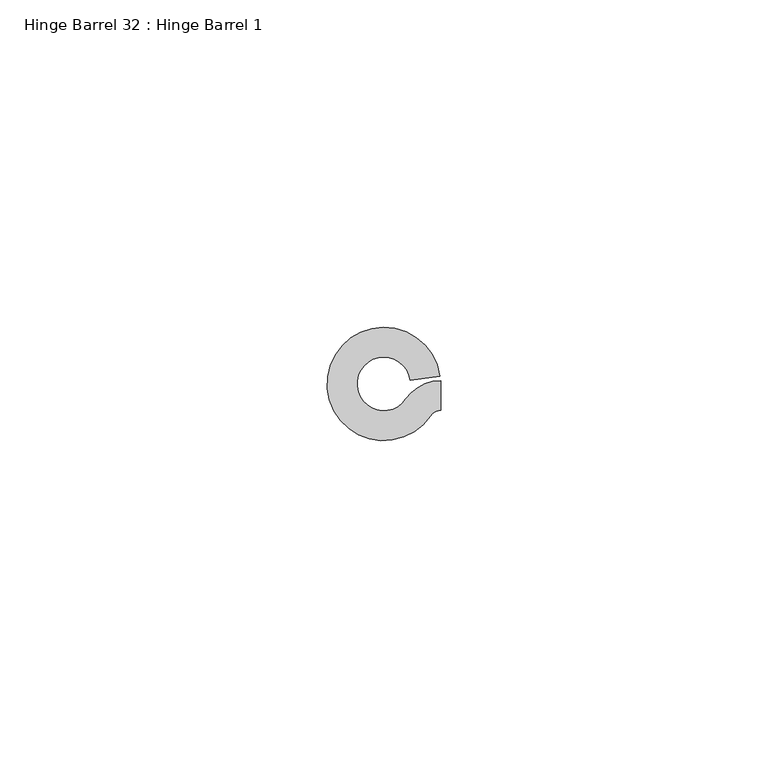
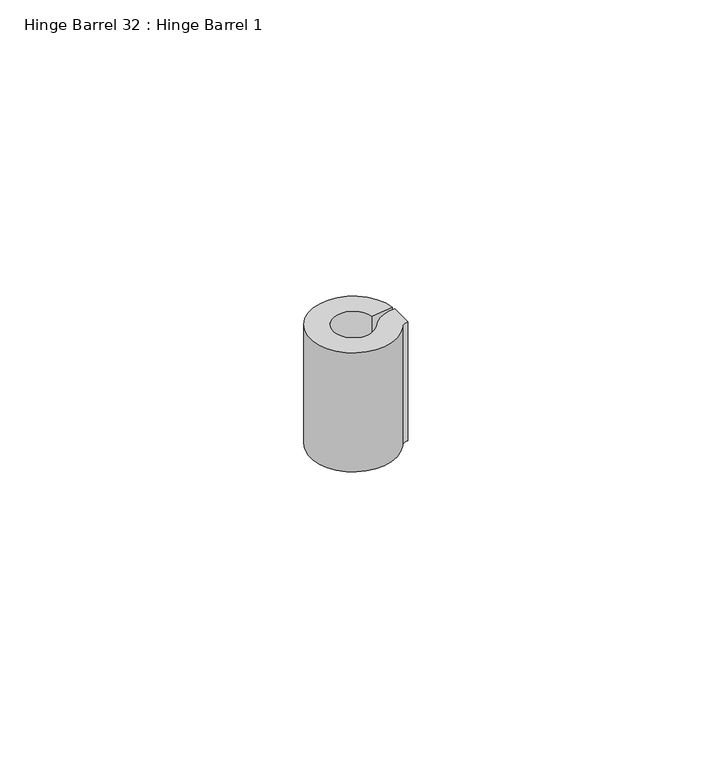
"""IFC4 building model written with IfcOpenShell, lengths in millimetres: proxy geometry, Hinge Barrel 32 : Hinge Barrel 1."""

import ifcopenshell
import ifcopenshell.guid

model = None  # the IFC model being written
_history = None  # IfcOwnerHistory: only IFC2X3 demands one
_inside = {}  # id of a spatial element -> (the spatial element, [elements in it])
_under = {}  # id of a project, library or spatial element -> (it, [spatial elements below it])
_declared = {}  # id of a project -> (the project, [libraries it declares])
_typed = {}  # id of a type object -> (the type object, [elements of that type])
_made_of = {}  # id of a material, layer set ... -> (it, [elements and type objects made of it])


def new_model(schema):
    """Start an empty IFC model of exactly this schema.

    Asked for "IFC4X3", IfcOpenShell would pick the latest addendum, in which some entities
    have other attributes; the version numbers below select the first issue.
    IFC2X3 requires an IfcOwnerHistory on every rooted entity: one is made here for all.
    """
    global model, _history
    if schema == "IFC4X3":
        model = ifcopenshell.file(schema_version=(4, 3, 0, 0))
    else:
        model = ifcopenshell.file(schema=schema)
    _inside.clear()
    _under.clear()
    _declared.clear()
    _typed.clear()
    _made_of.clear()
    _history = None
    if model.schema == "IFC2X3":
        org = make("IfcOrganization", Name="unknown")
        user = make(
            "IfcPersonAndOrganization",
            ThePerson=make("IfcPerson", FamilyName="unknown"),
            TheOrganization=org,
        )
        app = make(
            "IfcApplication",
            ApplicationDeveloper=org,
            Version="unknown",
            ApplicationFullName="unknown",
            ApplicationIdentifier="unknown",
        )
        _history = make(
            "IfcOwnerHistory",
            OwningUser=user,
            OwningApplication=app,
            ChangeAction="ADDED",
            CreationDate=0,
        )
    return model


def make(cls, **values):
    """One entity of the class cls with the attributes given. An attribute that is None is left unset."""
    return model.create_entity(
        cls, **{name: value for name, value in values.items() if value is not None}
    )


def rooted(cls, **values):
    """An entity with a GlobalId (a new one), such as an element, a storey or a relation."""
    return make(cls, GlobalId=ifcopenshell.guid.new(), OwnerHistory=_history, **values)


def si_unit(unit_type, name, prefix=None):
    """IfcSIUnit, for example si_unit("LENGTHUNIT", "METRE", prefix="MILLI")."""
    return make("IfcSIUnit", UnitType=unit_type, Prefix=prefix, Name=name)


def assignment(units):
    """IfcUnitAssignment: the units of a project."""
    return None if units is None else make("IfcUnitAssignment", Units=units)


def point(xyz):
    """IfcCartesianPoint."""
    return None if xyz is None else make("IfcCartesianPoint", Coordinates=xyz)


def direction(xyz):
    """IfcDirection."""
    return None if xyz is None else make("IfcDirection", DirectionRatios=xyz)


def frame(location, z_axis=None, x_axis=None):
    """IfcAxis2Placement3D, a coordinate frame: its origin and axes. An axis left out is left unset."""
    return make(
        "IfcAxis2Placement3D",
        Location=point(location),
        Axis=direction(z_axis),
        RefDirection=direction(x_axis),
    )


def frame_2d(location, x_axis=None):
    """IfcAxis2Placement2D, a coordinate frame in the plane: its origin and x axis."""
    return make(
        "IfcAxis2Placement2D", Location=point(location), RefDirection=direction(x_axis)
    )


def origin():
    """The frame at (0, 0, 0) with its axes left unset."""
    return frame((0.0, 0.0, 0.0))


def place(relative_to, where):
    """IfcLocalPlacement: puts the frame where relative to a parent placement (None: the world)."""
    return make(
        "IfcLocalPlacement", PlacementRelTo=relative_to, RelativePlacement=where
    )


def context(
    kind, dimensions, precision=None, world=None, true_north=None, identifier=None
):
    """IfcGeometricRepresentationContext, for example the 3D "Model" context."""
    return make(
        "IfcGeometricRepresentationContext",
        ContextIdentifier=identifier,
        ContextType=kind,
        CoordinateSpaceDimension=dimensions,
        Precision=precision,
        WorldCoordinateSystem=world,
        TrueNorth=true_north,
    )


def project(units=None, contexts=None):
    """IfcProject with its units and contexts."""
    return rooted(
        "IfcProject",
        Name="project",
        RepresentationContexts=contexts,
        UnitsInContext=assignment(units),
    )


def spatial(cls, under=None, at=None, **own):
    """A site, building, storey or space (cls), placed at a placement, below another one or the project."""
    s = rooted(cls, ObjectPlacement=at, **own)
    if under is not None:
        _under.setdefault(under.id(), (under, []))[1].append(s)
    return s


def polyline(points):
    """IfcPolyline through the points."""
    return make("IfcPolyline", Points=[point(p) for p in points])


def circle_curve(where, radius):
    """IfcCircle in the frame where."""
    return make("IfcCircle", Position=where, Radius=radius)


def trimmed(basis, trim1, trim2, sense, master):
    """IfcTrimmedCurve: the piece of a basis curve between two trims."""
    return make(
        "IfcTrimmedCurve",
        BasisCurve=basis,
        Trim1=trim1,
        Trim2=trim2,
        SenseAgreement=sense,
        MasterRepresentation=master,
    )


def segment(curve, same_sense, transition):
    """IfcCompositeCurveSegment."""
    return make(
        "IfcCompositeCurveSegment",
        Transition=transition,
        SameSense=same_sense,
        ParentCurve=curve,
    )


def composite_curve(segments, self_intersect=None):
    """IfcCompositeCurve: segments joined end to end."""
    return make("IfcCompositeCurve", Segments=segments, SelfIntersect=self_intersect)


def outline(outer, holes=None, kind="AREA"):
    """IfcArbitraryClosedProfileDef: a profile drawn as a closed curve; with holes, ...WithVoids."""
    if holes is None:
        return make("IfcArbitraryClosedProfileDef", ProfileType=kind, OuterCurve=outer)
    return make(
        "IfcArbitraryProfileDefWithVoids",
        ProfileType=kind,
        OuterCurve=outer,
        InnerCurves=holes,
    )


def extrude(swept, where, along, depth):
    """IfcExtrudedAreaSolid: the profile swept, set in the frame where, extruded along a direction by depth."""
    return make(
        "IfcExtrudedAreaSolid",
        SweptArea=swept,
        Position=where,
        ExtrudedDirection=direction(along),
        Depth=depth,
    )


def shape(context_of_items, identifier, shape_type, items):
    """IfcShapeRepresentation: the items that make up one representation, for example the "Body"."""
    return make(
        "IfcShapeRepresentation",
        ContextOfItems=context_of_items,
        RepresentationIdentifier=identifier,
        RepresentationType=shape_type,
        Items=items,
    )


def source(mapping_origin, context_of_items, identifier, shape_type, items):
    """IfcRepresentationMap: a shape defined once, which mapped items show again and again."""
    return make(
        "IfcRepresentationMap",
        MappingOrigin=mapping_origin,
        MappedRepresentation=shape(context_of_items, identifier, shape_type, items),
    )


def transform(
    local_origin,
    x_axis=None,
    y_axis=None,
    z_axis=None,
    scale=None,
    scale2=None,
    scale3=None,
    uniform=True,
):
    """IfcCartesianTransformationOperator3D, or its non-uniform kind. x_axis, y_axis, z_axis: its Axis1, 2, 3."""
    if uniform:
        return make(
            "IfcCartesianTransformationOperator3D",
            Axis1=direction(x_axis),
            Axis2=direction(y_axis),
            LocalOrigin=point(local_origin),
            Scale=scale,
            Axis3=direction(z_axis),
        )
    return make(
        "IfcCartesianTransformationOperator3DnonUniform",
        Axis1=direction(x_axis),
        Axis2=direction(y_axis),
        LocalOrigin=point(local_origin),
        Scale=scale,
        Axis3=direction(z_axis),
        Scale2=scale2,
        Scale3=scale3,
    )


def mapped(mapping_source, mapping_target):
    """IfcMappedItem: shows the shape of a source again, moved by a transform."""
    return make(
        "IfcMappedItem", MappingSource=mapping_source, MappingTarget=mapping_target
    )


def made_of(thing, what):
    """Note that an element or type object is made of a material, layer set ...; save() writes the relation."""
    if what is not None:
        _made_of.setdefault(what.id(), (what, []))[1].append(thing)
    return thing


def element(
    cls,
    number,
    at=None,
    inside=None,
    cuts=None,
    type_object=None,
    material=None,
    context=None,
    identifier="Body",
    shape_type=None,
    held_by="IfcProductDefinitionShape",
    body=None,
    shapes=None,
    **own,
):
    """One element of the class cls, such as IfcWall. Its Tag is "e" and its number.

    at: its placement. inside: the storey or other place that contains it. cuts: it is an
    opening in that element (IfcRelVoidsElement). A single representation is given by context,
    identifier, shape_type and body (its items); several are given by shapes. held_by: the class
    of the entity that holds the representations. save() writes the other relations.
    """
    e = rooted(cls, Tag="e%d" % number, ObjectPlacement=at, **own)
    if body is not None:
        shapes = [shape(context, identifier, shape_type, body)]
    if shapes is not None:
        e.Representation = make(held_by, Representations=shapes)
    if inside is not None:
        _inside.setdefault(inside.id(), (inside, []))[1].append(e)
    if cuts is not None:
        rooted(
            "IfcRelVoidsElement", RelatingBuildingElement=cuts, RelatedOpeningElement=e
        )
    if type_object is not None:
        _typed.setdefault(type_object.id(), (type_object, []))[1].append(e)
    return made_of(e, material)


def aggregate(whole, parts):
    """IfcRelAggregates: a whole, such as a stair, and the parts it consists of."""
    return rooted("IfcRelAggregates", RelatingObject=whole, RelatedObjects=parts)


def save(model, path):
    """Write the relations noted so far, then the file.

    IfcRelAggregates (storeys below a building ...), IfcRelContainedInSpatialStructure (elements
    in a storey), IfcRelDefinesByType, IfcRelAssociatesMaterial and IfcRelDeclares: one each for
    every whole, place, type object, material and project.
    """
    for whole, parts in _under.values():
        aggregate(whole, parts)
    for where, things in _inside.values():
        rooted(
            "IfcRelContainedInSpatialStructure",
            RelatedElements=things,
            RelatingStructure=where,
        )
    for kind, things in _typed.values():
        rooted("IfcRelDefinesByType", RelatedObjects=things, RelatingType=kind)
    for what, things in _made_of.values():
        rooted("IfcRelAssociatesMaterial", RelatedObjects=things, RelatingMaterial=what)
    for by, libraries in _declared.values():
        rooted("IfcRelDeclares", RelatingContext=by, RelatedDefinitions=libraries)
    model.write(path)


def hinge_barrel_32_hinge_barrel_1_17cad03c(model_context):
    return source(origin(), model_context, "Body", "SweptSolid", [
        extrude(outline(composite_curve([segment(trimmed(circle_curve(frame_2d((587327.8245257, -533990.5568067)), 6.4044851), [point((587322.5194669, -533986.9688017))], [point((587327.8245257, -533984.1523216))], False, "CARTESIAN"), True, "CONTINUOUS"), segment(polyline([(587327.8245257, -533984.1523216), (587327.8245257, -533988.7163841)]), True, "CONTINUOUS"), segment(trimmed(circle_curve(frame_2d((587327.8245257, -533990.5568067)), 1.8404226), [point((587327.8245257, -533988.7163841))], [point((587326.3000393, -533989.5257409))], True, "CARTESIAN"), True, "CONTINUOUS"), segment(trimmed(circle_curve(frame_2d((587319.1320739, -533984.6777841)), 8.6534625), [point((587326.3000393, -533989.5257409))], [point((587327.7022899, -533983.4803654))], False, "CARTESIAN"), True, "CONTINUOUS"), segment(polyline([(587327.7022899, -533983.4803654), (587323.1821338, -533984.1119153)]), True, "CONTINUOUS"), segment(trimmed(circle_curve(frame_2d((587319.1320739, -533984.6777841)), 4.0894), [point((587323.1821338, -533984.1119153))], [point((587322.5194669, -533986.9688017))], True, "CARTESIAN"), True, "CONTINUOUS")], self_intersect=False)), frame((0.0, 0.0, 1149.35), z_axis=(0.0, 0.0, 1.0), x_axis=(1.0, 0.0, 0.0)), (0.0, 0.0, 1.0), 25.4),
    ])


if __name__ == "__main__":
    model = new_model("IFC4")
    model_context = context("Model", 3, world=origin())
    ifc_project = project(units=[si_unit("LENGTHUNIT", "METRE", prefix="MILLI")], contexts=[model_context])
    site = spatial("IfcSite", under=ifc_project)
    building = spatial("IfcBuilding", under=site)
    placement = place(None, origin())
    hinge_barrel_32_hinge_barrel_1_shape = hinge_barrel_32_hinge_barrel_1_17cad03c(model_context)
    element("IfcBuildingElementProxy", 1, Name="Hinge Barrel 32 : Hinge Barrel 1", ObjectType="Hinge Barrel 32 : Hinge Barrel 1", at=placement, inside=building, context=model_context, shape_type="MappedRepresentation", body=[
        mapped(hinge_barrel_32_hinge_barrel_1_shape, transform((0.0, 0.0, 0.0), x_axis=(1.0, 0.0, 0.0), y_axis=(0.0, 1.0, 0.0), z_axis=(0.0, 0.0, 1.0))),
    ])
    save(model, "model.ifc")

# Revit data of these elements
# Element 1 (IfcBuildingElementProxy, "Hinge Barrel 32 : Hinge Barrel 1")
#   Materials on its faces: "6\"X6\" WELD-ON STL BUTT HINGE"
# Materials
#   "6\"X6\" WELD-ON STL BUTT HINGE": class "Metal", colour RGB 189 187 185, transparency 0, Description = "Carbon steel", Cost = 0
